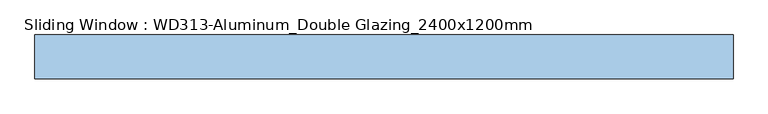
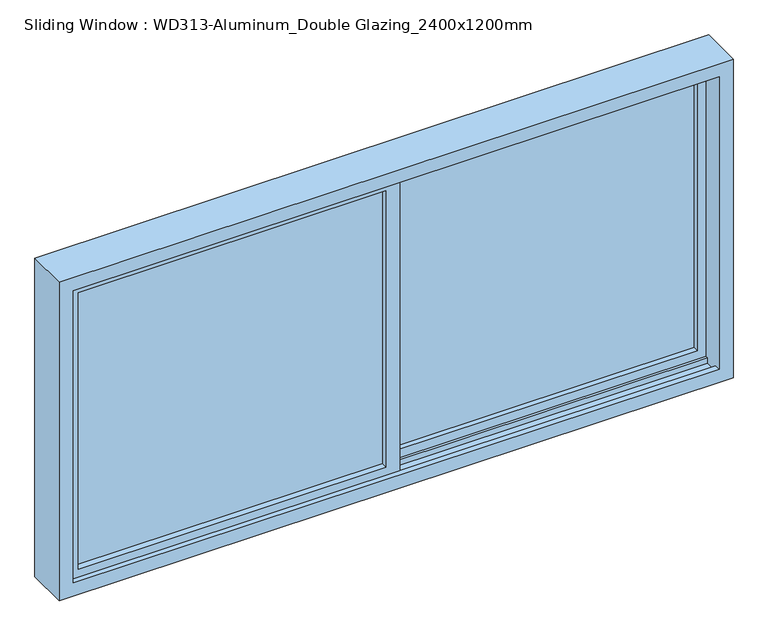
"""IFC4 building model written with IfcOpenShell, lengths in millimetres: window geometry, Sliding Window : WD313-Aluminum_Double Glazing_2400x1200mm."""

from ifc_helpers import new_model, si_unit, frame, origin, place, context, project, spatial, polyline, outline, extrude, faceted_brep, source, transform, mapped, element, save


def sliding_window_wd313_aluminum_double_glazing_2400x1200mm_47b363be(model_context):
    return source(origin(), model_context, "Body", "SolidModel", [
        extrude(outline(polyline([(1120.0, 27.5), (25.0, 27.5), (25.0, 32.5), (1120.0, 32.5), (1120.0, 27.5)])), frame((0.0, 0.0, 680.0), z_axis=(0.0, 0.0, 1.0), x_axis=(1.0, 0.0, 0.0)), (0.0, 0.0, 1.0), 1040.0),
        extrude(outline(polyline([(-25.0, -32.5), (-1120.0, -32.5), (-1120.0, -27.5), (-25.0, -27.5), (-25.0, -32.5)])), frame((0.0, 0.0, 680.0), z_axis=(0.0, 0.0, 1.0), x_axis=(1.0, 0.0, 0.0)), (0.0, 0.0, 1.0), 1040.0),
        extrude(outline(polyline([(630.0, -1170.0), (630.0, 25.0), (1770.0, 25.0), (1770.0, -1170.0), (630.0, -1170.0)]), holes=[polyline([(1720.0, -1120.0), (1720.0, -25.0), (680.0, -25.0), (680.0, -1120.0), (1720.0, -1120.0)])]), frame((0.0, -55.0, 0.0), z_axis=(0.0, 1.0, 0.0), x_axis=(0.0, 0.0, 1.0)), (0.0, 0.0, 1.0), 47.5),
        extrude(outline(polyline([(630.0, -25.0), (630.0, 1170.0), (1770.0, 1170.0), (1770.0, -25.0), (630.0, -25.0)]), holes=[polyline([(1720.0, 25.0), (1720.0, 1120.0), (680.0, 1120.0), (680.0, 25.0), (1720.0, 25.0)])]), frame((0.0, 7.5, 0.0), z_axis=(0.0, 1.0, 0.0), x_axis=(0.0, 0.0, 1.0)), (0.0, 0.0, 1.0), 45.0),
        faceted_brep([(-1200.0, 75.0, 1800.0), (-1200.0, 75.0, 600.0), (-1200.0, -75.0, 600.0), (-1200.0, -75.0, 1800.0), (1200.0, 75.0, 1800.0), (1200.0, 75.0, 600.0), (1150.0, 75.0, 650.0), (1150.0, 75.0, 1750.0), (-1150.0, 75.0, 1750.0), (-1150.0, 75.0, 650.0), (1200.0, -75.0, 600.0), (1200.0, -75.0, 1800.0), (-1150.0, -75.0, 1750.0), (1150.0, -75.0, 1750.0), (1150.0, -75.0, 650.0), (-1150.0, -75.0, 650.0), (1150.0, 55.0, 650.0), (1150.0, 55.0, 1750.0), (-1150.0, 55.0, 1750.0), (-1150.0, 55.0, 1770.0), (-1150.0, 5.0, 1770.0), (-1150.0, 5.0, 1750.0), (-1150.0, -5.0, 1750.0), (-1150.0, -5.0, 650.0), (-1150.0, 5.0, 650.0), (-1150.0, 5.0, 630.0), (-1150.0, 55.0, 630.0), (-1150.0, 55.0, 650.0), (1150.0, -5.0, 650.0), (1150.0, 5.0, 650.0), (1150.0, -5.0, 630.0), (1150.0, -55.0, 630.0), (1150.0, -55.0, 650.0), (1150.0, -55.0, 1750.0), (1150.0, -55.0, 1770.0), (1150.0, -5.0, 1770.0), (1150.0, -5.0, 1750.0), (1150.0, 5.0, 1750.0), (1170.0, 5.0, 1770.0), (1170.0, 5.0, 630.0), (-1170.0, -5.0, 1770.0), (-1170.0, -5.0, 630.0), (1170.0, 55.0, 1770.0), (1170.0, 55.0, 630.0), (-1170.0, -55.0, 630.0), (-1150.0, -55.0, 1750.0), (-1150.0, -55.0, 650.0), (-1170.0, -55.0, 1770.0)], [[[0, 1, 2, 3]], [[4, 5, 1, 0], [6, 7, 8, 9]], [[1, 5, 10, 2]], [[10, 11, 3, 2], [12, 13, 14, 15]], [[7, 6, 16, 17]], [[9, 8, 18, 19, 20, 21, 22, 23, 24, 25, 26, 27]], [[16, 6, 9, 27]], [[5, 4, 11, 10]], [[28, 29, 24, 23]], [[28, 30, 31, 32, 14, 13, 33, 34, 35, 36, 37, 29]], [[29, 37, 21, 20, 38, 39, 25, 24]], [[40, 41, 30, 28, 23, 22, 36, 35]], [[39, 38, 42, 43]], [[39, 43, 26, 25]], [[43, 42, 19, 18, 17, 16, 27, 26]], [[41, 44, 31, 30]], [[45, 46, 32, 31, 44, 47, 34, 33]], [[46, 15, 14, 32]], [[12, 15, 46, 45]], [[47, 44, 41, 40]], [[3, 11, 4, 0]], [[37, 36, 22, 21]], [[42, 38, 20, 19]], [[7, 17, 18, 8]], [[12, 45, 33, 13]], [[47, 40, 35, 34]]]),
    ])


if __name__ == "__main__":
    model = new_model("IFC4")
    model_context = context("Model", 3, world=origin())
    ifc_project = project(units=[si_unit("LENGTHUNIT", "METRE", prefix="MILLI")], contexts=[model_context])
    site = spatial("IfcSite", under=ifc_project)
    building = spatial("IfcBuilding", under=site)
    placement = place(None, origin())
    sliding_window_wd313_aluminum_double_glazing_2400x1200mm_shape = sliding_window_wd313_aluminum_double_glazing_2400x1200mm_47b363be(model_context)
    element("IfcWindow", 1, ObjectType="Sliding Window : WD313-Aluminum_Double Glazing_2400x1200mm", at=placement, inside=building, context=model_context, shape_type="MappedRepresentation", body=[
        mapped(sliding_window_wd313_aluminum_double_glazing_2400x1200mm_shape, transform((0.0, 0.0, 0.0), x_axis=(1.0, 0.0, 0.0), y_axis=(0.0, 1.0, 0.0), z_axis=(0.0, 0.0, 1.0))),
    ])
    save(model, "model.ifc")

# Revit data of these elements
# Type "Sliding Window : WD313-Aluminum_Double Glazing_2400x1200mm"
#   Type Mark = "PW"
#   Analytic Construction = "<None>"
#   창 두께 = 150 mm
#   Visual Light Transmittance = 0.9
#   Thermal Resistance (R) = 0.271106 (m²·K)/W
#   Solar Heat Gain Coefficient = 0.78
#   Height = 1200 mm
#   Heat Transfer Coefficient (U) = 3.6886 W/(m²·K)
#   기본 씰 높이 = 600 mm
#   Width = 2400 mm
#   Define Thermal Properties by = 1
#   창 패널 = AW1 창 패널
#   창 프레임 = A04AQ127-00002_Aluminum Window_None FP
#   Description = (empty or 0)
#   Construction Type Id = ""
#   Wall Closure = (empty or 0)
# Element 1 (IfcWindow, "Sliding Window : WD313-Aluminum_Double Glazing_2400x1200mm")
#   Materials on its faces: "A04AQ127-00002_Aluminum Window_None FP", "AW1 창 패널"
# Materials
#   "AW1 창 패널": class "유리", colour RGB 0 0 255, transparency 0.75
#   "A04AQ127-00002_Aluminum Window_None FP": class "금속", colour RGB 247 247 247, transparency 0, W00) Work Master Code = "A04AQ127-00002", W01) Work Master_Lv1 = "Finishing Work", W02) Work Master_Lv2 = "Door & Window Work", W03) Work Master_Spec.1 = "Aluminum Window", W04) Work Master_Spec.2 = "Fire Protective Rating: N/A", W05) Work Master_Spec.3 = "w/ Hardware & Accessories", Cost = 0
